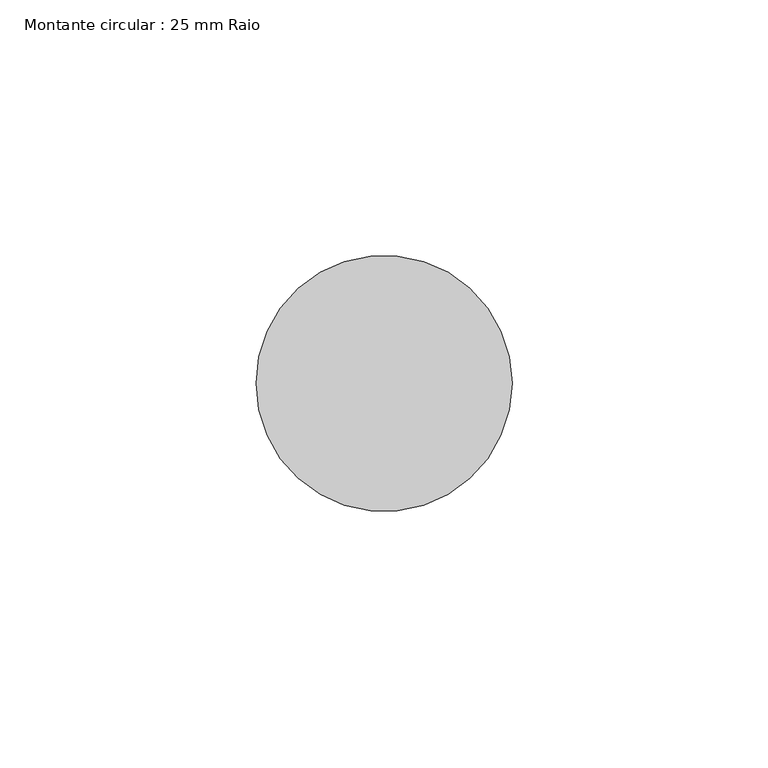
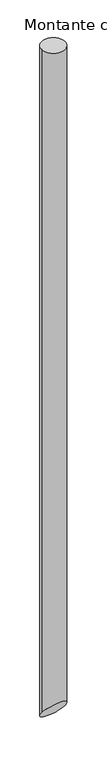
"""IFC4 building model written with IfcOpenShell, lengths in millimetres: member geometry, Montante circular : 25 mm Raio."""

import ifcopenshell
import ifcopenshell.guid

model = None  # the IFC model being written
_history = None  # IfcOwnerHistory: only IFC2X3 demands one
_inside = {}  # id of a spatial element -> (the spatial element, [elements in it])
_under = {}  # id of a project, library or spatial element -> (it, [spatial elements below it])
_declared = {}  # id of a project -> (the project, [libraries it declares])
_typed = {}  # id of a type object -> (the type object, [elements of that type])
_made_of = {}  # id of a material, layer set ... -> (it, [elements and type objects made of it])


def new_model(schema):
    """Start an empty IFC model of exactly this schema.

    Asked for "IFC4X3", IfcOpenShell would pick the latest addendum, in which some entities
    have other attributes; the version numbers below select the first issue.
    IFC2X3 requires an IfcOwnerHistory on every rooted entity: one is made here for all.
    """
    global model, _history
    if schema == "IFC4X3":
        model = ifcopenshell.file(schema_version=(4, 3, 0, 0))
    else:
        model = ifcopenshell.file(schema=schema)
    _inside.clear()
    _under.clear()
    _declared.clear()
    _typed.clear()
    _made_of.clear()
    _history = None
    if model.schema == "IFC2X3":
        org = make("IfcOrganization", Name="unknown")
        user = make(
            "IfcPersonAndOrganization",
            ThePerson=make("IfcPerson", FamilyName="unknown"),
            TheOrganization=org,
        )
        app = make(
            "IfcApplication",
            ApplicationDeveloper=org,
            Version="unknown",
            ApplicationFullName="unknown",
            ApplicationIdentifier="unknown",
        )
        _history = make(
            "IfcOwnerHistory",
            OwningUser=user,
            OwningApplication=app,
            ChangeAction="ADDED",
            CreationDate=0,
        )
    return model


def make(cls, **values):
    """One entity of the class cls with the attributes given. An attribute that is None is left unset."""
    return model.create_entity(
        cls, **{name: value for name, value in values.items() if value is not None}
    )


def rooted(cls, **values):
    """An entity with a GlobalId (a new one), such as an element, a storey or a relation."""
    return make(cls, GlobalId=ifcopenshell.guid.new(), OwnerHistory=_history, **values)


def si_unit(unit_type, name, prefix=None):
    """IfcSIUnit, for example si_unit("LENGTHUNIT", "METRE", prefix="MILLI")."""
    return make("IfcSIUnit", UnitType=unit_type, Prefix=prefix, Name=name)


def assignment(units):
    """IfcUnitAssignment: the units of a project."""
    return None if units is None else make("IfcUnitAssignment", Units=units)


def point(xyz):
    """IfcCartesianPoint."""
    return None if xyz is None else make("IfcCartesianPoint", Coordinates=xyz)


def direction(xyz):
    """IfcDirection."""
    return None if xyz is None else make("IfcDirection", DirectionRatios=xyz)


def frame(location, z_axis=None, x_axis=None):
    """IfcAxis2Placement3D, a coordinate frame: its origin and axes. An axis left out is left unset."""
    return make(
        "IfcAxis2Placement3D",
        Location=point(location),
        Axis=direction(z_axis),
        RefDirection=direction(x_axis),
    )


def origin():
    """The frame at (0, 0, 0) with its axes left unset."""
    return frame((0.0, 0.0, 0.0))


def place(relative_to, where):
    """IfcLocalPlacement: puts the frame where relative to a parent placement (None: the world)."""
    return make(
        "IfcLocalPlacement", PlacementRelTo=relative_to, RelativePlacement=where
    )


def context(
    kind, dimensions, precision=None, world=None, true_north=None, identifier=None
):
    """IfcGeometricRepresentationContext, for example the 3D "Model" context."""
    return make(
        "IfcGeometricRepresentationContext",
        ContextIdentifier=identifier,
        ContextType=kind,
        CoordinateSpaceDimension=dimensions,
        Precision=precision,
        WorldCoordinateSystem=world,
        TrueNorth=true_north,
    )


def project(units=None, contexts=None):
    """IfcProject with its units and contexts."""
    return rooted(
        "IfcProject",
        Name="project",
        RepresentationContexts=contexts,
        UnitsInContext=assignment(units),
    )


def spatial(cls, under=None, at=None, **own):
    """A site, building, storey or space (cls), placed at a placement, below another one or the project."""
    s = rooted(cls, ObjectPlacement=at, **own)
    if under is not None:
        _under.setdefault(under.id(), (under, []))[1].append(s)
    return s


def circle_curve(where, radius):
    """IfcCircle in the frame where."""
    return make("IfcCircle", Position=where, Radius=radius)


def ellipse_curve(where, semi_axis1, semi_axis2):
    """IfcEllipse in the frame where."""
    return make(
        "IfcEllipse", Position=where, SemiAxis1=semi_axis1, SemiAxis2=semi_axis2
    )


def shape(context_of_items, identifier, shape_type, items):
    """IfcShapeRepresentation: the items that make up one representation, for example the "Body"."""
    return make(
        "IfcShapeRepresentation",
        ContextOfItems=context_of_items,
        RepresentationIdentifier=identifier,
        RepresentationType=shape_type,
        Items=items,
    )


def source(mapping_origin, context_of_items, identifier, shape_type, items):
    """IfcRepresentationMap: a shape defined once, which mapped items show again and again."""
    return make(
        "IfcRepresentationMap",
        MappingOrigin=mapping_origin,
        MappedRepresentation=shape(context_of_items, identifier, shape_type, items),
    )


def transform(
    local_origin,
    x_axis=None,
    y_axis=None,
    z_axis=None,
    scale=None,
    scale2=None,
    scale3=None,
    uniform=True,
):
    """IfcCartesianTransformationOperator3D, or its non-uniform kind. x_axis, y_axis, z_axis: its Axis1, 2, 3."""
    if uniform:
        return make(
            "IfcCartesianTransformationOperator3D",
            Axis1=direction(x_axis),
            Axis2=direction(y_axis),
            LocalOrigin=point(local_origin),
            Scale=scale,
            Axis3=direction(z_axis),
        )
    return make(
        "IfcCartesianTransformationOperator3DnonUniform",
        Axis1=direction(x_axis),
        Axis2=direction(y_axis),
        LocalOrigin=point(local_origin),
        Scale=scale,
        Axis3=direction(z_axis),
        Scale2=scale2,
        Scale3=scale3,
    )


def mapped(mapping_source, mapping_target):
    """IfcMappedItem: shows the shape of a source again, moved by a transform."""
    return make(
        "IfcMappedItem", MappingSource=mapping_source, MappingTarget=mapping_target
    )


def made_of(thing, what):
    """Note that an element or type object is made of a material, layer set ...; save() writes the relation."""
    if what is not None:
        _made_of.setdefault(what.id(), (what, []))[1].append(thing)
    return thing


def element(
    cls,
    number,
    at=None,
    inside=None,
    cuts=None,
    type_object=None,
    material=None,
    context=None,
    identifier="Body",
    shape_type=None,
    held_by="IfcProductDefinitionShape",
    body=None,
    shapes=None,
    **own,
):
    """One element of the class cls, such as IfcWall. Its Tag is "e" and its number.

    at: its placement. inside: the storey or other place that contains it. cuts: it is an
    opening in that element (IfcRelVoidsElement). A single representation is given by context,
    identifier, shape_type and body (its items); several are given by shapes. held_by: the class
    of the entity that holds the representations. save() writes the other relations.
    """
    e = rooted(cls, Tag="e%d" % number, ObjectPlacement=at, **own)
    if body is not None:
        shapes = [shape(context, identifier, shape_type, body)]
    if shapes is not None:
        e.Representation = make(held_by, Representations=shapes)
    if inside is not None:
        _inside.setdefault(inside.id(), (inside, []))[1].append(e)
    if cuts is not None:
        rooted(
            "IfcRelVoidsElement", RelatingBuildingElement=cuts, RelatedOpeningElement=e
        )
    if type_object is not None:
        _typed.setdefault(type_object.id(), (type_object, []))[1].append(e)
    return made_of(e, material)


def aggregate(whole, parts):
    """IfcRelAggregates: a whole, such as a stair, and the parts it consists of."""
    return rooted("IfcRelAggregates", RelatingObject=whole, RelatedObjects=parts)


def save(model, path):
    """Write the relations noted so far, then the file.

    IfcRelAggregates (storeys below a building ...), IfcRelContainedInSpatialStructure (elements
    in a storey), IfcRelDefinesByType, IfcRelAssociatesMaterial and IfcRelDeclares: one each for
    every whole, place, type object, material and project.
    """
    for whole, parts in _under.values():
        aggregate(whole, parts)
    for where, things in _inside.values():
        rooted(
            "IfcRelContainedInSpatialStructure",
            RelatedElements=things,
            RelatingStructure=where,
        )
    for kind, things in _typed.values():
        rooted("IfcRelDefinesByType", RelatedObjects=things, RelatingType=kind)
    for what, things in _made_of.values():
        rooted("IfcRelAssociatesMaterial", RelatedObjects=things, RelatingMaterial=what)
    for by, libraries in _declared.values():
        rooted("IfcRelDeclares", RelatingContext=by, RelatedDefinitions=libraries)
    model.write(path)


def plane_surface(at):
    """IfcPlane: the flat surface through the origin of the frame at, square to its z axis."""
    return make("IfcPlane", Position=at)


def cylinder_surface(at, radius):
    """IfcCylindricalSurface: all points at the distance radius from the z axis of the frame at."""
    return make("IfcCylindricalSurface", Position=at, Radius=radius)


def advanced_brep(points, edges, surfaces, faces):
    """IfcAdvancedBrep: a solid bounded by faces that lie on surfaces and meet in shared edges.

    An edge is (start, end): straight between two places in points (the first is 0);
    or (start, end, curve); or (start, end, curve, False) where it runs against its curve.
    A face is (place in surfaces, loops), or (place, loops, False) where it looks against
    its surface's normal. A loop lists edges by number (the first is 1), with a minus sign
    where the edge is run from its end to its start. The first loop is the outer one.
    """
    corners = [point(p) for p in points]
    vertices = [make("IfcVertexPoint", VertexGeometry=c) for c in corners]
    made = []
    for start, end, *more in edges:
        made.append(
            make(
                "IfcEdgeCurve",
                EdgeStart=vertices[start],
                EdgeEnd=vertices[end],
                EdgeGeometry=more[0] if more else make("IfcPolyline", Points=[corners[start], corners[end]]),
                SameSense=more[1] if len(more) > 1 else True,
            )
        )
    hull = []
    for where, loops, *sense in faces:
        bounds = []
        for j, loop in enumerate(loops):
            ring = [make("IfcOrientedEdge", EdgeElement=made[abs(k) - 1], Orientation=k > 0) for k in loop]
            bounds.append(
                make(
                    "IfcFaceOuterBound" if j == 0 else "IfcFaceBound",
                    Bound=make("IfcEdgeLoop", EdgeList=ring),
                    Orientation=True,
                )
            )
        hull.append(make("IfcAdvancedFace", Bounds=bounds, FaceSurface=surfaces[where], SameSense=sense[0] if sense else True))
    return make("IfcAdvancedBrep", Outer=make("IfcClosedShell", CfsFaces=hull))


def montante_circular_25_mm_raio_72299cf2(model_context):
    return source(origin(), model_context, "Body", "AdvancedBrep", [
        advanced_brep(
        [(0.0, 0.0, 0.0), (-50.0, 0.0, 0.0), (0.0, 0.0, -1500.0), (-50.0, 0.0, -1500.0)],
        [
            (0, 1, circle_curve(frame((-25.0, 0.0, 0.0), z_axis=(0.0, 0.0, 1.0), x_axis=(1.0, 0.0, 0.0)), 25.0)),
            (1, 0, circle_curve(frame((-25.0, 0.0, 0.0), z_axis=(0.0, 0.0, 1.0), x_axis=(1.0, 0.0, 0.0)), 25.0)),
            (0, 2),
            (2, 3, ellipse_curve(frame((-25.0, 0.0, -1500.0), z_axis=(0.0, 0.7735779641603617, 0.6337011388387355), x_axis=(0.0, -0.6337011388387355, 0.7735779641603615)), 39.4507734, 25.0)),
            (3, 1),
            (3, 2, ellipse_curve(frame((-25.0, 0.0, -1500.0), z_axis=(0.0, 0.7735779641603617, 0.6337011388387355), x_axis=(0.0, -0.6337011388387355, 0.7735779641603615)), 39.4507734, 25.0)),
        ],
        [
            plane_surface(frame((0.0, -50.0, 0.0), z_axis=(0.0, 0.0, 1.0), x_axis=(-1.0, 0.0, 0.0))),
            cylinder_surface(frame((-25.0, 0.0, 0.0), z_axis=(0.0, 0.0, 1.0), x_axis=(1.0, 0.0, 0.0)), 25.0),
            plane_surface(frame((304.8, 0.0, -1500.0), z_axis=(0.0, -0.7735779641603617, -0.6337011388387355), x_axis=(0.0, -0.6337011388387355, 0.7735779641603617))),
        ],
        [
            (0, [[1, 2]]),
            (1, [[-1, 3, 4, 5]]),
            (1, [[-2, -5, 6, -3]]),
            (2, [[-6, -4]]),
        ],
    ),
    ])


if __name__ == "__main__":
    model = new_model("IFC4")
    model_context = context("Model", 3, world=origin())
    ifc_project = project(units=[si_unit("LENGTHUNIT", "METRE", prefix="MILLI")], contexts=[model_context])
    site = spatial("IfcSite", under=ifc_project)
    building = spatial("IfcBuilding", under=site)
    placement = place(None, origin())
    montante_circular_25_mm_raio_shape = montante_circular_25_mm_raio_72299cf2(model_context)
    element("IfcMember", 1, ObjectType="Montante circular : 25 mm Raio", at=placement, inside=building, context=model_context, shape_type="MappedRepresentation", body=[
        mapped(montante_circular_25_mm_raio_shape, transform((0.0, 0.0, 0.0), x_axis=(1.0, 0.0, 0.0), y_axis=(0.0, 1.0, 0.0), z_axis=(0.0, 0.0, 1.0))),
    ])
    save(model, "model.ifc")

# Revit data of these elements
# Type "Montante circular : 25 mm Raio"
#   built-in parameter 1007350 = 0.082021 (stored number, unit not read)
# Element 1 (IfcMember, "Montante circular : 25 mm Raio")
#   Materials on its faces: "Alumín."
# Materials
#   "Alumín.": class "Metal", colour RGB 247 247 247, transparency 0, Description = "Alumín. 6061", Cost = 0
